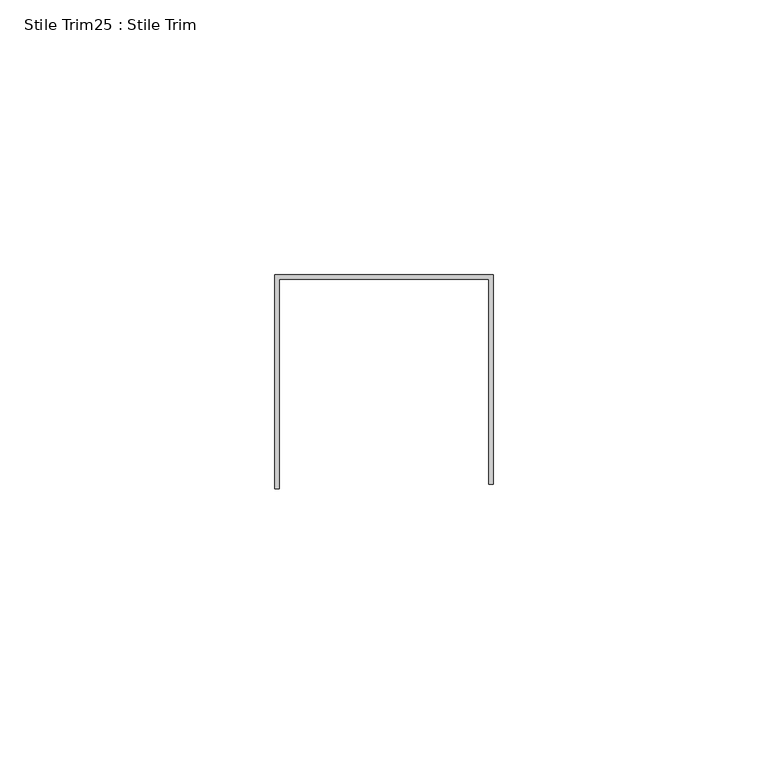
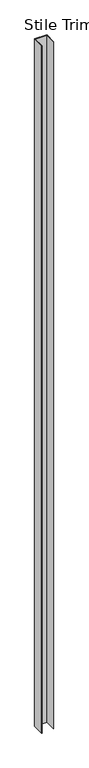
"""IFC4 building model written with IfcOpenShell, lengths in millimetres: proxy geometry, Stile Trim25 : Stile Trim."""

from ifc_helpers import new_model, si_unit, frame, origin, place, context, project, spatial, polyline, outline, extrude, source, transform, mapped, element, save


def stile_trim25_stile_trim_18cce888(model_context):
    return source(origin(), model_context, "Body", "SweptSolid", [
        extrude(outline(polyline([(587327.0060739, -535207.1289841), (587366.6808739, -535207.1289841), (587366.6808739, -535245.2289841), (587365.8934739, -535245.2289841), (587365.8934739, -535207.9163841), (587327.7934739, -535207.9163841), (587327.7934739, -535246.0163841), (587327.0060739, -535246.0163841), (587327.0060739, -535207.1289841)])), frame((0.0, 0.0, 50.8), z_axis=(0.0, 0.0, 1.0), x_axis=(1.0, 0.0, 0.0)), (0.0, 0.0, 1.0), 2350.3929688),
    ])


if __name__ == "__main__":
    model = new_model("IFC4")
    model_context = context("Model", 3, world=origin())
    ifc_project = project(units=[si_unit("LENGTHUNIT", "METRE", prefix="MILLI")], contexts=[model_context])
    site = spatial("IfcSite", under=ifc_project)
    building = spatial("IfcBuilding", under=site)
    placement = place(None, origin())
    stile_trim25_stile_trim_shape = stile_trim25_stile_trim_18cce888(model_context)
    element("IfcBuildingElementProxy", 1, Name="Stile Trim25 : Stile Trim", ObjectType="Stile Trim25 : Stile Trim", at=placement, inside=building, context=model_context, shape_type="MappedRepresentation", body=[
        mapped(stile_trim25_stile_trim_shape, transform((0.0, 0.0, 0.0), x_axis=(1.0, 0.0, 0.0), y_axis=(0.0, 1.0, 0.0), z_axis=(0.0, 0.0, 1.0))),
    ])
    save(model, "model.ifc")

# Revit data of these elements
# Element 1 (IfcBuildingElementProxy, "Stile Trim25 : Stile Trim")
#   Materials on its faces: "EDGE TRIM BY MTL PANEL MFR."
# Materials
#   "EDGE TRIM BY MTL PANEL MFR.": class "Generic", colour RGB 239 242 240, transparency 0, Cost = 0
